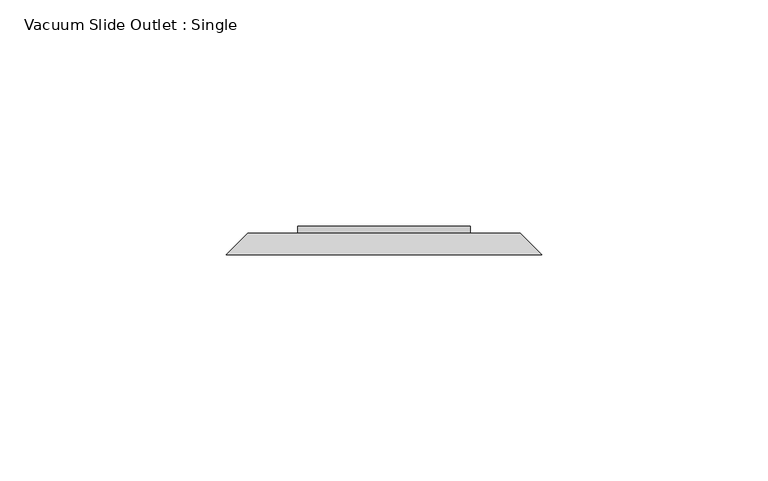
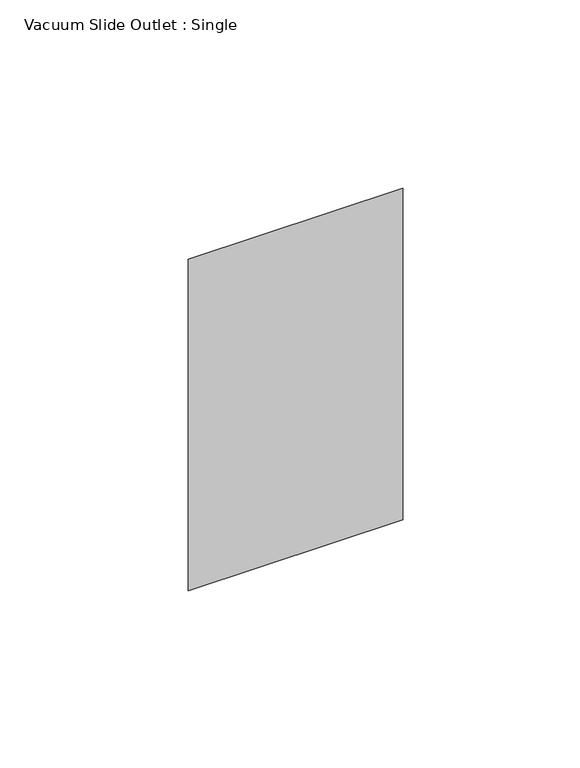
"""IFC4 building model written with IfcOpenShell, lengths in millimetres: proxy geometry, Vacuum Slide Outlet : Single."""

import ifcopenshell
import ifcopenshell.guid

model = None  # the IFC model being written
_history = None  # IfcOwnerHistory: only IFC2X3 demands one
_inside = {}  # id of a spatial element -> (the spatial element, [elements in it])
_under = {}  # id of a project, library or spatial element -> (it, [spatial elements below it])
_declared = {}  # id of a project -> (the project, [libraries it declares])
_typed = {}  # id of a type object -> (the type object, [elements of that type])
_made_of = {}  # id of a material, layer set ... -> (it, [elements and type objects made of it])


def new_model(schema):
    """Start an empty IFC model of exactly this schema.

    Asked for "IFC4X3", IfcOpenShell would pick the latest addendum, in which some entities
    have other attributes; the version numbers below select the first issue.
    IFC2X3 requires an IfcOwnerHistory on every rooted entity: one is made here for all.
    """
    global model, _history
    if schema == "IFC4X3":
        model = ifcopenshell.file(schema_version=(4, 3, 0, 0))
    else:
        model = ifcopenshell.file(schema=schema)
    _inside.clear()
    _under.clear()
    _declared.clear()
    _typed.clear()
    _made_of.clear()
    _history = None
    if model.schema == "IFC2X3":
        org = make("IfcOrganization", Name="unknown")
        user = make(
            "IfcPersonAndOrganization",
            ThePerson=make("IfcPerson", FamilyName="unknown"),
            TheOrganization=org,
        )
        app = make(
            "IfcApplication",
            ApplicationDeveloper=org,
            Version="unknown",
            ApplicationFullName="unknown",
            ApplicationIdentifier="unknown",
        )
        _history = make(
            "IfcOwnerHistory",
            OwningUser=user,
            OwningApplication=app,
            ChangeAction="ADDED",
            CreationDate=0,
        )
    return model


def make(cls, **values):
    """One entity of the class cls with the attributes given. An attribute that is None is left unset."""
    return model.create_entity(
        cls, **{name: value for name, value in values.items() if value is not None}
    )


def rooted(cls, **values):
    """An entity with a GlobalId (a new one), such as an element, a storey or a relation."""
    return make(cls, GlobalId=ifcopenshell.guid.new(), OwnerHistory=_history, **values)


def si_unit(unit_type, name, prefix=None):
    """IfcSIUnit, for example si_unit("LENGTHUNIT", "METRE", prefix="MILLI")."""
    return make("IfcSIUnit", UnitType=unit_type, Prefix=prefix, Name=name)


def assignment(units):
    """IfcUnitAssignment: the units of a project."""
    return None if units is None else make("IfcUnitAssignment", Units=units)


def point(xyz):
    """IfcCartesianPoint."""
    return None if xyz is None else make("IfcCartesianPoint", Coordinates=xyz)


def direction(xyz):
    """IfcDirection."""
    return None if xyz is None else make("IfcDirection", DirectionRatios=xyz)


def frame(location, z_axis=None, x_axis=None):
    """IfcAxis2Placement3D, a coordinate frame: its origin and axes. An axis left out is left unset."""
    return make(
        "IfcAxis2Placement3D",
        Location=point(location),
        Axis=direction(z_axis),
        RefDirection=direction(x_axis),
    )


def origin():
    """The frame at (0, 0, 0) with its axes left unset."""
    return frame((0.0, 0.0, 0.0))


def place(relative_to, where):
    """IfcLocalPlacement: puts the frame where relative to a parent placement (None: the world)."""
    return make(
        "IfcLocalPlacement", PlacementRelTo=relative_to, RelativePlacement=where
    )


def context(
    kind, dimensions, precision=None, world=None, true_north=None, identifier=None
):
    """IfcGeometricRepresentationContext, for example the 3D "Model" context."""
    return make(
        "IfcGeometricRepresentationContext",
        ContextIdentifier=identifier,
        ContextType=kind,
        CoordinateSpaceDimension=dimensions,
        Precision=precision,
        WorldCoordinateSystem=world,
        TrueNorth=true_north,
    )


def project(units=None, contexts=None):
    """IfcProject with its units and contexts."""
    return rooted(
        "IfcProject",
        Name="project",
        RepresentationContexts=contexts,
        UnitsInContext=assignment(units),
    )


def spatial(cls, under=None, at=None, **own):
    """A site, building, storey or space (cls), placed at a placement, below another one or the project."""
    s = rooted(cls, ObjectPlacement=at, **own)
    if under is not None:
        _under.setdefault(under.id(), (under, []))[1].append(s)
    return s


def polyline(points):
    """IfcPolyline through the points."""
    return make("IfcPolyline", Points=[point(p) for p in points])


def outline(outer, holes=None, kind="AREA"):
    """IfcArbitraryClosedProfileDef: a profile drawn as a closed curve; with holes, ...WithVoids."""
    if holes is None:
        return make("IfcArbitraryClosedProfileDef", ProfileType=kind, OuterCurve=outer)
    return make(
        "IfcArbitraryProfileDefWithVoids",
        ProfileType=kind,
        OuterCurve=outer,
        InnerCurves=holes,
    )


def extrude(swept, where, along, depth):
    """IfcExtrudedAreaSolid: the profile swept, set in the frame where, extruded along a direction by depth."""
    return make(
        "IfcExtrudedAreaSolid",
        SweptArea=swept,
        Position=where,
        ExtrudedDirection=direction(along),
        Depth=depth,
    )


def faces_of(points, faces, orient=None, outer=None):
    """IfcFace entities. A face is a list of loops; a loop is a list of indices into points, from 0.

    orient and outer hold one flag for each loop. By default every Orientation is true, the
    first loop of a face is its IfcFaceOuterBound and the others are IfcFaceBound.
    """
    made = []
    for i, loops in enumerate(faces):
        bounds = []
        for j, loop in enumerate(loops):
            is_outer = j == 0 if outer is None else outer[i][j]
            bounds.append(
                make(
                    "IfcFaceOuterBound" if is_outer else "IfcFaceBound",
                    Bound=make("IfcPolyLoop", Polygon=[points[k] for k in loop]),
                    Orientation=True if orient is None else orient[i][j],
                )
            )
        made.append(make("IfcFace", Bounds=bounds))
    return made


def faceted_brep(points, faces, orient=None, outer=None, voids=None):
    """IfcFacetedBrep: a solid bounded by flat faces; with voids (closed shells), ...WithVoids."""
    shared = [point(p) for p in points]
    hull = make("IfcClosedShell", CfsFaces=faces_of(shared, faces, orient, outer))
    if voids is None:
        return make("IfcFacetedBrep", Outer=hull)
    return make(
        "IfcFacetedBrepWithVoids",
        Outer=hull,
        Voids=[
            make(cls, CfsFaces=faces_of(shared, fs, o, b)) for cls, fs, o, b in voids
        ],
    )


def shape(context_of_items, identifier, shape_type, items):
    """IfcShapeRepresentation: the items that make up one representation, for example the "Body"."""
    return make(
        "IfcShapeRepresentation",
        ContextOfItems=context_of_items,
        RepresentationIdentifier=identifier,
        RepresentationType=shape_type,
        Items=items,
    )


def source(mapping_origin, context_of_items, identifier, shape_type, items):
    """IfcRepresentationMap: a shape defined once, which mapped items show again and again."""
    return make(
        "IfcRepresentationMap",
        MappingOrigin=mapping_origin,
        MappedRepresentation=shape(context_of_items, identifier, shape_type, items),
    )


def transform(
    local_origin,
    x_axis=None,
    y_axis=None,
    z_axis=None,
    scale=None,
    scale2=None,
    scale3=None,
    uniform=True,
):
    """IfcCartesianTransformationOperator3D, or its non-uniform kind. x_axis, y_axis, z_axis: its Axis1, 2, 3."""
    if uniform:
        return make(
            "IfcCartesianTransformationOperator3D",
            Axis1=direction(x_axis),
            Axis2=direction(y_axis),
            LocalOrigin=point(local_origin),
            Scale=scale,
            Axis3=direction(z_axis),
        )
    return make(
        "IfcCartesianTransformationOperator3DnonUniform",
        Axis1=direction(x_axis),
        Axis2=direction(y_axis),
        LocalOrigin=point(local_origin),
        Scale=scale,
        Axis3=direction(z_axis),
        Scale2=scale2,
        Scale3=scale3,
    )


def mapped(mapping_source, mapping_target):
    """IfcMappedItem: shows the shape of a source again, moved by a transform."""
    return make(
        "IfcMappedItem", MappingSource=mapping_source, MappingTarget=mapping_target
    )


def made_of(thing, what):
    """Note that an element or type object is made of a material, layer set ...; save() writes the relation."""
    if what is not None:
        _made_of.setdefault(what.id(), (what, []))[1].append(thing)
    return thing


def element(
    cls,
    number,
    at=None,
    inside=None,
    cuts=None,
    type_object=None,
    material=None,
    context=None,
    identifier="Body",
    shape_type=None,
    held_by="IfcProductDefinitionShape",
    body=None,
    shapes=None,
    **own,
):
    """One element of the class cls, such as IfcWall. Its Tag is "e" and its number.

    at: its placement. inside: the storey or other place that contains it. cuts: it is an
    opening in that element (IfcRelVoidsElement). A single representation is given by context,
    identifier, shape_type and body (its items); several are given by shapes. held_by: the class
    of the entity that holds the representations. save() writes the other relations.
    """
    e = rooted(cls, Tag="e%d" % number, ObjectPlacement=at, **own)
    if body is not None:
        shapes = [shape(context, identifier, shape_type, body)]
    if shapes is not None:
        e.Representation = make(held_by, Representations=shapes)
    if inside is not None:
        _inside.setdefault(inside.id(), (inside, []))[1].append(e)
    if cuts is not None:
        rooted(
            "IfcRelVoidsElement", RelatingBuildingElement=cuts, RelatedOpeningElement=e
        )
    if type_object is not None:
        _typed.setdefault(type_object.id(), (type_object, []))[1].append(e)
    return made_of(e, material)


def aggregate(whole, parts):
    """IfcRelAggregates: a whole, such as a stair, and the parts it consists of."""
    return rooted("IfcRelAggregates", RelatingObject=whole, RelatedObjects=parts)


def save(model, path):
    """Write the relations noted so far, then the file.

    IfcRelAggregates (storeys below a building ...), IfcRelContainedInSpatialStructure (elements
    in a storey), IfcRelDefinesByType, IfcRelAssociatesMaterial and IfcRelDeclares: one each for
    every whole, place, type object, material and project.
    """
    for whole, parts in _under.values():
        aggregate(whole, parts)
    for where, things in _inside.values():
        rooted(
            "IfcRelContainedInSpatialStructure",
            RelatedElements=things,
            RelatingStructure=where,
        )
    for kind, things in _typed.values():
        rooted("IfcRelDefinesByType", RelatedObjects=things, RelatingType=kind)
    for what, things in _made_of.values():
        rooted("IfcRelAssociatesMaterial", RelatedObjects=things, RelatingMaterial=what)
    for by, libraries in _declared.values():
        rooted("IfcRelDeclares", RelatingContext=by, RelatedDefinitions=libraries)
    model.write(path)


def vacuum_slide_outlet_single_fa60efc4(model_context):
    return source(origin(), model_context, "Body", "SolidModel", [
        extrude(outline(polyline([(19.05, 66.675), (-19.05, 66.675), (-19.05, 68.2625), (19.05, 68.2625), (19.05, 66.675)])), frame((0.0, 0.0, 869.95), z_axis=(0.0, 0.0, 1.0), x_axis=(1.0, 0.0, 0.0)), (0.0, 0.0, 1.0), 88.9),
        faceted_brep([(-30.1625, 66.675, 966.7875), (30.1625, 66.675, 966.7875), (30.1625, 66.675, 862.0125), (-30.1625, 66.675, 862.0125), (-34.925, 61.9125, 971.55), (-34.925, 61.9125, 857.25), (34.925, 61.9125, 857.25), (34.925, 61.9125, 971.55)], [[[0, 1, 2, 3]], [[4, 5, 6, 7]], [[4, 7, 1, 0]], [[7, 6, 2, 1]], [[6, 5, 3, 2]], [[5, 4, 0, 3]]]),
    ])


if __name__ == "__main__":
    model = new_model("IFC4")
    model_context = context("Model", 3, world=origin())
    ifc_project = project(units=[si_unit("LENGTHUNIT", "METRE", prefix="MILLI")], contexts=[model_context])
    site = spatial("IfcSite", under=ifc_project)
    building = spatial("IfcBuilding", under=site)
    placement = place(None, origin())
    vacuum_slide_outlet_single_shape = vacuum_slide_outlet_single_fa60efc4(model_context)
    element("IfcBuildingElementProxy", 1, Name="Vacuum Slide Outlet : Single", ObjectType="Vacuum Slide Outlet : Single", at=placement, inside=building, context=model_context, shape_type="MappedRepresentation", body=[
        mapped(vacuum_slide_outlet_single_shape, transform((0.0, 0.0, 0.0), x_axis=(1.0, 0.0, 0.0), y_axis=(0.0, 1.0, 0.0), z_axis=(0.0, 0.0, 1.0))),
    ])
    save(model, "model.ifc")

# Revit data of these elements
# Type "Vacuum Slide Outlet : Single"
#   Label [instance default] = "PM"
#   Width = 0' - 2 3/4"
#   Placement Height = 3' - 0"
#   Height = 0' - 4 1/2"
#   Material = Plastic - White
#   Keynote = ""
# Element 1 (IfcBuildingElementProxy, "Vacuum Slide Outlet : Single")
#   Materials on its faces: "Plastic - White"
# Materials
#   "Plastic - White": class "Unassigned", colour RGB 249 249 249, transparency 0
